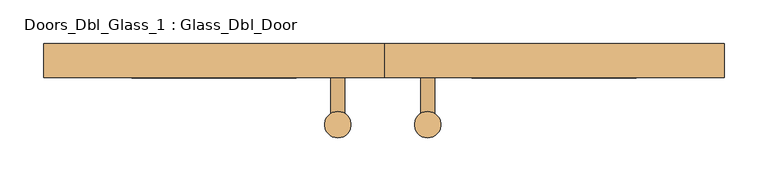
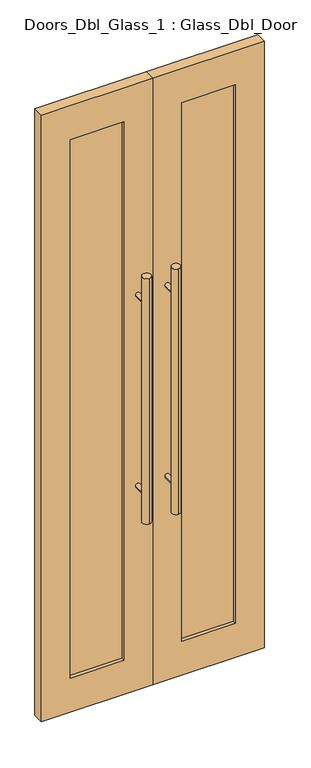
"""IFC4 building model written with IfcOpenShell, lengths in millimetres: door geometry, Doors_Dbl_Glass_1 : Glass_Dbl_Door."""

import ifcopenshell
import ifcopenshell.guid

model = None  # the IFC model being written
_history = None  # IfcOwnerHistory: only IFC2X3 demands one
_inside = {}  # id of a spatial element -> (the spatial element, [elements in it])
_under = {}  # id of a project, library or spatial element -> (it, [spatial elements below it])
_declared = {}  # id of a project -> (the project, [libraries it declares])
_typed = {}  # id of a type object -> (the type object, [elements of that type])
_made_of = {}  # id of a material, layer set ... -> (it, [elements and type objects made of it])


def new_model(schema):
    """Start an empty IFC model of exactly this schema.

    Asked for "IFC4X3", IfcOpenShell would pick the latest addendum, in which some entities
    have other attributes; the version numbers below select the first issue.
    IFC2X3 requires an IfcOwnerHistory on every rooted entity: one is made here for all.
    """
    global model, _history
    if schema == "IFC4X3":
        model = ifcopenshell.file(schema_version=(4, 3, 0, 0))
    else:
        model = ifcopenshell.file(schema=schema)
    _inside.clear()
    _under.clear()
    _declared.clear()
    _typed.clear()
    _made_of.clear()
    _history = None
    if model.schema == "IFC2X3":
        org = make("IfcOrganization", Name="unknown")
        user = make(
            "IfcPersonAndOrganization",
            ThePerson=make("IfcPerson", FamilyName="unknown"),
            TheOrganization=org,
        )
        app = make(
            "IfcApplication",
            ApplicationDeveloper=org,
            Version="unknown",
            ApplicationFullName="unknown",
            ApplicationIdentifier="unknown",
        )
        _history = make(
            "IfcOwnerHistory",
            OwningUser=user,
            OwningApplication=app,
            ChangeAction="ADDED",
            CreationDate=0,
        )
    return model


def make(cls, **values):
    """One entity of the class cls with the attributes given. An attribute that is None is left unset."""
    return model.create_entity(
        cls, **{name: value for name, value in values.items() if value is not None}
    )


def rooted(cls, **values):
    """An entity with a GlobalId (a new one), such as an element, a storey or a relation."""
    return make(cls, GlobalId=ifcopenshell.guid.new(), OwnerHistory=_history, **values)


def si_unit(unit_type, name, prefix=None):
    """IfcSIUnit, for example si_unit("LENGTHUNIT", "METRE", prefix="MILLI")."""
    return make("IfcSIUnit", UnitType=unit_type, Prefix=prefix, Name=name)


def assignment(units):
    """IfcUnitAssignment: the units of a project."""
    return None if units is None else make("IfcUnitAssignment", Units=units)


def point(xyz):
    """IfcCartesianPoint."""
    return None if xyz is None else make("IfcCartesianPoint", Coordinates=xyz)


def direction(xyz):
    """IfcDirection."""
    return None if xyz is None else make("IfcDirection", DirectionRatios=xyz)


def frame(location, z_axis=None, x_axis=None):
    """IfcAxis2Placement3D, a coordinate frame: its origin and axes. An axis left out is left unset."""
    return make(
        "IfcAxis2Placement3D",
        Location=point(location),
        Axis=direction(z_axis),
        RefDirection=direction(x_axis),
    )


def frame_2d(location, x_axis=None):
    """IfcAxis2Placement2D, a coordinate frame in the plane: its origin and x axis."""
    return make(
        "IfcAxis2Placement2D", Location=point(location), RefDirection=direction(x_axis)
    )


def origin():
    """The frame at (0, 0, 0) with its axes left unset."""
    return frame((0.0, 0.0, 0.0))


def place(relative_to, where):
    """IfcLocalPlacement: puts the frame where relative to a parent placement (None: the world)."""
    return make(
        "IfcLocalPlacement", PlacementRelTo=relative_to, RelativePlacement=where
    )


def context(
    kind, dimensions, precision=None, world=None, true_north=None, identifier=None
):
    """IfcGeometricRepresentationContext, for example the 3D "Model" context."""
    return make(
        "IfcGeometricRepresentationContext",
        ContextIdentifier=identifier,
        ContextType=kind,
        CoordinateSpaceDimension=dimensions,
        Precision=precision,
        WorldCoordinateSystem=world,
        TrueNorth=true_north,
    )


def project(units=None, contexts=None):
    """IfcProject with its units and contexts."""
    return rooted(
        "IfcProject",
        Name="project",
        RepresentationContexts=contexts,
        UnitsInContext=assignment(units),
    )


def spatial(cls, under=None, at=None, **own):
    """A site, building, storey or space (cls), placed at a placement, below another one or the project."""
    s = rooted(cls, ObjectPlacement=at, **own)
    if under is not None:
        _under.setdefault(under.id(), (under, []))[1].append(s)
    return s


def polyline(points):
    """IfcPolyline through the points."""
    return make("IfcPolyline", Points=[point(p) for p in points])


def circle_curve(where, radius):
    """IfcCircle in the frame where."""
    return make("IfcCircle", Position=where, Radius=radius)


def trimmed(basis, trim1, trim2, sense, master):
    """IfcTrimmedCurve: the piece of a basis curve between two trims."""
    return make(
        "IfcTrimmedCurve",
        BasisCurve=basis,
        Trim1=trim1,
        Trim2=trim2,
        SenseAgreement=sense,
        MasterRepresentation=master,
    )


def segment(curve, same_sense, transition):
    """IfcCompositeCurveSegment."""
    return make(
        "IfcCompositeCurveSegment",
        Transition=transition,
        SameSense=same_sense,
        ParentCurve=curve,
    )


def composite_curve(segments, self_intersect=None):
    """IfcCompositeCurve: segments joined end to end."""
    return make("IfcCompositeCurve", Segments=segments, SelfIntersect=self_intersect)


def outline(outer, holes=None, kind="AREA"):
    """IfcArbitraryClosedProfileDef: a profile drawn as a closed curve; with holes, ...WithVoids."""
    if holes is None:
        return make("IfcArbitraryClosedProfileDef", ProfileType=kind, OuterCurve=outer)
    return make(
        "IfcArbitraryProfileDefWithVoids",
        ProfileType=kind,
        OuterCurve=outer,
        InnerCurves=holes,
    )


def extrude(swept, where, along, depth):
    """IfcExtrudedAreaSolid: the profile swept, set in the frame where, extruded along a direction by depth."""
    return make(
        "IfcExtrudedAreaSolid",
        SweptArea=swept,
        Position=where,
        ExtrudedDirection=direction(along),
        Depth=depth,
    )


def shape(context_of_items, identifier, shape_type, items):
    """IfcShapeRepresentation: the items that make up one representation, for example the "Body"."""
    return make(
        "IfcShapeRepresentation",
        ContextOfItems=context_of_items,
        RepresentationIdentifier=identifier,
        RepresentationType=shape_type,
        Items=items,
    )


def source(mapping_origin, context_of_items, identifier, shape_type, items):
    """IfcRepresentationMap: a shape defined once, which mapped items show again and again."""
    return make(
        "IfcRepresentationMap",
        MappingOrigin=mapping_origin,
        MappedRepresentation=shape(context_of_items, identifier, shape_type, items),
    )


def transform(
    local_origin,
    x_axis=None,
    y_axis=None,
    z_axis=None,
    scale=None,
    scale2=None,
    scale3=None,
    uniform=True,
):
    """IfcCartesianTransformationOperator3D, or its non-uniform kind. x_axis, y_axis, z_axis: its Axis1, 2, 3."""
    if uniform:
        return make(
            "IfcCartesianTransformationOperator3D",
            Axis1=direction(x_axis),
            Axis2=direction(y_axis),
            LocalOrigin=point(local_origin),
            Scale=scale,
            Axis3=direction(z_axis),
        )
    return make(
        "IfcCartesianTransformationOperator3DnonUniform",
        Axis1=direction(x_axis),
        Axis2=direction(y_axis),
        LocalOrigin=point(local_origin),
        Scale=scale,
        Axis3=direction(z_axis),
        Scale2=scale2,
        Scale3=scale3,
    )


def mapped(mapping_source, mapping_target):
    """IfcMappedItem: shows the shape of a source again, moved by a transform."""
    return make(
        "IfcMappedItem", MappingSource=mapping_source, MappingTarget=mapping_target
    )


def made_of(thing, what):
    """Note that an element or type object is made of a material, layer set ...; save() writes the relation."""
    if what is not None:
        _made_of.setdefault(what.id(), (what, []))[1].append(thing)
    return thing


def element(
    cls,
    number,
    at=None,
    inside=None,
    cuts=None,
    type_object=None,
    material=None,
    context=None,
    identifier="Body",
    shape_type=None,
    held_by="IfcProductDefinitionShape",
    body=None,
    shapes=None,
    **own,
):
    """One element of the class cls, such as IfcWall. Its Tag is "e" and its number.

    at: its placement. inside: the storey or other place that contains it. cuts: it is an
    opening in that element (IfcRelVoidsElement). A single representation is given by context,
    identifier, shape_type and body (its items); several are given by shapes. held_by: the class
    of the entity that holds the representations. save() writes the other relations.
    """
    e = rooted(cls, Tag="e%d" % number, ObjectPlacement=at, **own)
    if body is not None:
        shapes = [shape(context, identifier, shape_type, body)]
    if shapes is not None:
        e.Representation = make(held_by, Representations=shapes)
    if inside is not None:
        _inside.setdefault(inside.id(), (inside, []))[1].append(e)
    if cuts is not None:
        rooted(
            "IfcRelVoidsElement", RelatingBuildingElement=cuts, RelatedOpeningElement=e
        )
    if type_object is not None:
        _typed.setdefault(type_object.id(), (type_object, []))[1].append(e)
    return made_of(e, material)


def aggregate(whole, parts):
    """IfcRelAggregates: a whole, such as a stair, and the parts it consists of."""
    return rooted("IfcRelAggregates", RelatingObject=whole, RelatedObjects=parts)


def save(model, path):
    """Write the relations noted so far, then the file.

    IfcRelAggregates (storeys below a building ...), IfcRelContainedInSpatialStructure (elements
    in a storey), IfcRelDefinesByType, IfcRelAssociatesMaterial and IfcRelDeclares: one each for
    every whole, place, type object, material and project.
    """
    for whole, parts in _under.values():
        aggregate(whole, parts)
    for where, things in _inside.values():
        rooted(
            "IfcRelContainedInSpatialStructure",
            RelatedElements=things,
            RelatingStructure=where,
        )
    for kind, things in _typed.values():
        rooted("IfcRelDefinesByType", RelatedObjects=things, RelatingType=kind)
    for what, things in _made_of.values():
        rooted("IfcRelAssociatesMaterial", RelatedObjects=things, RelatingMaterial=what)
    for by, libraries in _declared.values():
        rooted("IfcRelDeclares", RelatingContext=by, RelatedDefinitions=libraries)
    model.write(path)


def doors_dbl_glass_1_glass_dbl_door_a30122f7(model_context):
    return source(origin(), model_context, "Body", "SweptSolid", [
        extrude(outline(composite_curve([segment(trimmed(circle_curve(frame_2d((49.6069979, -116.0715804)), 15.0), [point((49.6069979, -101.0715804))], [point((49.6069979, -131.0715804))], False, "CARTESIAN"), True, "CONTINUOUS"), segment(trimmed(circle_curve(frame_2d((49.6069979, -116.0715804)), 15.0), [point((49.6069979, -131.0715804))], [point((49.6069979, -101.0715804))], False, "CARTESIAN"), True, "CONTINUOUS")], self_intersect=False)), frame((0.0, 0.0, 650.0), z_axis=(0.0, 0.0, 1.0), x_axis=(1.0, 0.0, 0.0)), (0.0, 0.0, 1.0), 900.0),
        extrude(outline(composite_curve([segment(trimmed(circle_curve(frame_2d((-52.537897, -116.0715804)), 15.0), [point((-52.537897, -101.0715804))], [point((-52.537897, -131.0715804))], False, "CARTESIAN"), True, "CONTINUOUS"), segment(trimmed(circle_curve(frame_2d((-52.537897, -116.0715804)), 15.0), [point((-52.537897, -131.0715804))], [point((-52.537897, -101.0715804))], False, "CARTESIAN"), True, "CONTINUOUS")], self_intersect=False)), frame((0.0, 0.0, 650.0), z_axis=(0.0, 0.0, 1.0), x_axis=(1.0, 0.0, 0.0)), (0.0, 0.0, 1.0), 900.0),
        extrude(outline(composite_curve([segment(trimmed(circle_curve(frame_2d((750.0, 49.6069979)), 8.0), [point((750.0, 57.6069979))], [point((750.0, 41.6069979))], False, "CARTESIAN"), True, "CONTINUOUS"), segment(trimmed(circle_curve(frame_2d((750.0, 49.6069979)), 8.0), [point((750.0, 41.6069979))], [point((750.0, 57.6069979))], False, "CARTESIAN"), True, "CONTINUOUS")], self_intersect=False)), frame((0.0, -116.0715804, 0.0), z_axis=(0.0, 1.0, 0.0), x_axis=(0.0, 0.0, 1.0)), (0.0, 0.0, 1.0), 53.4927248),
        extrude(outline(composite_curve([segment(trimmed(circle_curve(frame_2d((750.0, -52.537897)), 8.0), [point((750.0, -44.537897))], [point((750.0, -60.537897))], False, "CARTESIAN"), True, "CONTINUOUS"), segment(trimmed(circle_curve(frame_2d((750.0, -52.537897)), 8.0), [point((750.0, -60.537897))], [point((750.0, -44.537897))], False, "CARTESIAN"), True, "CONTINUOUS")], self_intersect=False)), frame((0.0, -116.0715804, 0.0), z_axis=(0.0, 1.0, 0.0), x_axis=(0.0, 0.0, 1.0)), (0.0, 0.0, 1.0), 53.4927248),
        extrude(outline(composite_curve([segment(trimmed(circle_curve(frame_2d((1450.0, 49.6069979)), 8.0), [point((1450.0, 57.6069979))], [point((1450.0, 41.6069979))], False, "CARTESIAN"), True, "CONTINUOUS"), segment(trimmed(circle_curve(frame_2d((1450.0, 49.6069979)), 8.0), [point((1450.0, 41.6069979))], [point((1450.0, 57.6069979))], False, "CARTESIAN"), True, "CONTINUOUS")], self_intersect=False)), frame((0.0, -116.0715804, 0.0), z_axis=(0.0, 1.0, 0.0), x_axis=(0.0, 0.0, 1.0)), (0.0, 0.0, 1.0), 53.4927248),
        extrude(outline(composite_curve([segment(trimmed(circle_curve(frame_2d((1450.0, -52.537897)), 8.0), [point((1450.0, -44.537897))], [point((1450.0, -60.537897))], False, "CARTESIAN"), True, "CONTINUOUS"), segment(trimmed(circle_curve(frame_2d((1450.0, -52.537897)), 8.0), [point((1450.0, -60.537897))], [point((1450.0, -44.537897))], False, "CARTESIAN"), True, "CONTINUOUS")], self_intersect=False)), frame((0.0, -116.0715804, 0.0), z_axis=(0.0, 1.0, 0.0), x_axis=(0.0, 0.0, 1.0)), (0.0, 0.0, 1.0), 53.4927248),
        extrude(outline(polyline([(2225.0, -386.7001888), (0.0, -386.7001888), (0.0, 0.0), (2225.0, 0.0), (2225.0, -386.7001888)]), holes=[polyline([(2100.0, -286.7001888), (2100.0, -100.0), (125.0, -100.0), (125.0, -286.7001888), (2100.0, -286.7001888)])]), frame((0.0, -62.5788556, 0.0), z_axis=(0.0, 1.0, 0.0), x_axis=(0.0, 0.0, 1.0)), (0.0, 0.0, 1.0), 38.5435966),
        extrude(outline(polyline([(2225.0, 0.0), (0.0, 0.0), (0.0, 386.7001888), (2225.0, 386.7001888), (2225.0, 0.0)]), holes=[polyline([(2100.0, 100.0), (2100.0, 286.7001888), (125.0, 286.7001888), (125.0, 100.0), (2100.0, 100.0)])]), frame((0.0, -62.5788556, 0.0), z_axis=(0.0, 1.0, 0.0), x_axis=(0.0, 0.0, 1.0)), (0.0, 0.0, 1.0), 38.5435966),
        extrude(outline(polyline([(-100.0, -38.0), (-100.0, -50.0), (-286.7001888, -50.0), (-286.7001888, -38.0), (-100.0, -38.0)])), frame((0.0, 0.0, 125.0), z_axis=(0.0, 0.0, 1.0), x_axis=(1.0, 0.0, 0.0)), (0.0, 0.0, 1.0), 1975.0),
        extrude(outline(polyline([(286.7001888, -38.0), (286.7001888, -50.0), (100.0, -50.0), (100.0, -38.0), (286.7001888, -38.0)])), frame((0.0, 0.0, 125.0), z_axis=(0.0, 0.0, 1.0), x_axis=(1.0, 0.0, 0.0)), (0.0, 0.0, 1.0), 1975.0),
    ])


if __name__ == "__main__":
    model = new_model("IFC4")
    model_context = context("Model", 3, world=origin())
    ifc_project = project(units=[si_unit("LENGTHUNIT", "METRE", prefix="MILLI")], contexts=[model_context])
    site = spatial("IfcSite", under=ifc_project)
    building = spatial("IfcBuilding", under=site)
    placement = place(None, origin())
    doors_dbl_glass_1_glass_dbl_door_shape = doors_dbl_glass_1_glass_dbl_door_a30122f7(model_context)
    element("IfcDoor", 1, ObjectType="Doors_Dbl_Glass_1 : Glass_Dbl_Door", at=placement, inside=building, context=model_context, shape_type="MappedRepresentation", body=[
        mapped(doors_dbl_glass_1_glass_dbl_door_shape, transform((0.0, 0.0, 0.0), x_axis=(1.0, 0.0, 0.0), y_axis=(0.0, 1.0, 0.0), z_axis=(0.0, 0.0, 1.0))),
    ])
    save(model, "model.ifc")

# Revit data of these elements
# Type "Doors_Dbl_Glass_1 : Glass_Dbl_Door"
#   Type Mark = "47"
#   Construction Type Id = "GSP4R"
#   Analytic Construction = "1/8 in Pilkington single glazing"
#   Visual Light Transmittance = 0.9
#   Stile Shutting = 100 mm
#   Stile Hanging = 100 mm
#   Stile - Top Rail = 125 mm
#   Stile - Bottom Rail = 125 mm
#   Solar Heat Gain Coefficient = 0.78
#   Offset = 50 mm
#   Heat Transfer Coefficient (U) = 3.6886 W/(m²·K)
#   Glass Thickness = 12 mm
#   Material Ironmongery = Metal - Aluminum
#   Material Door = Metal - Aluminum
#   Material Glass = Glass
#   Function = (empty or 0)
# Element 1 (IfcDoor, "Doors_Dbl_Glass_1 : Glass_Dbl_Door")
#   Materials on its faces: "Metal - Aluminum", "Glass"
# Materials
#   "Metal - Aluminum": class "Metal", colour RGB 247 247 247, transparency 0
#   "Glass": class "Glass", colour RGB 0 128 192, transparency 0.9, Description = "Soda Lime Glass", Cost = 0
